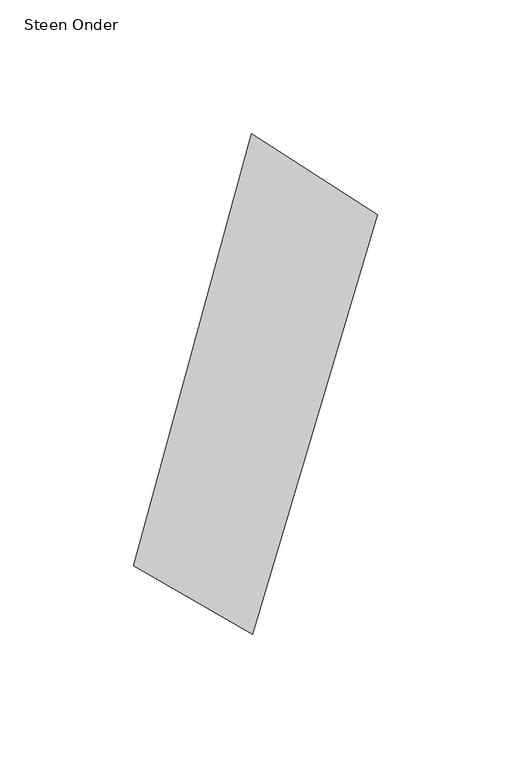
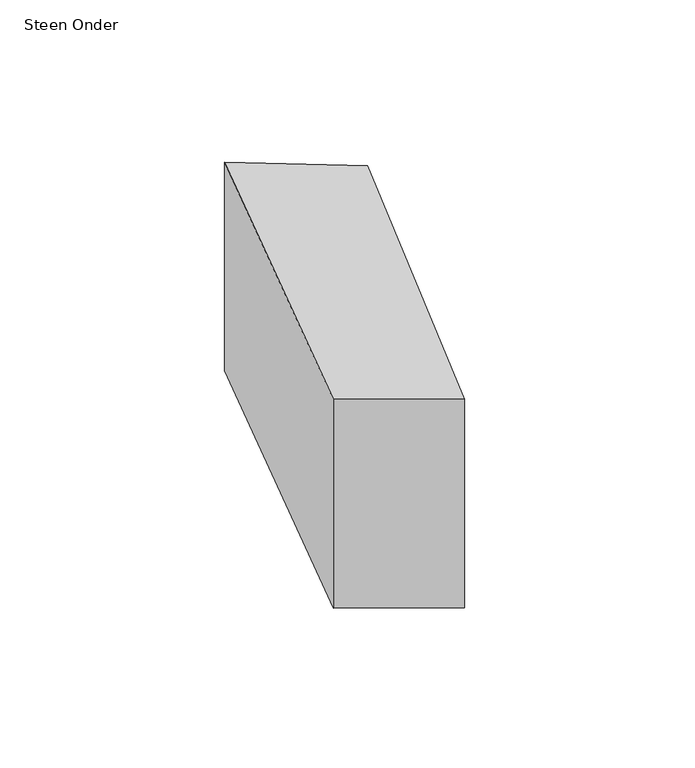
"""IFC4 building model written with IfcOpenShell, lengths in millimetres: proxy geometry, 00_GMA_steen_versie_4 : Steen Onder."""

import ifcopenshell
import ifcopenshell.guid

model = None  # the IFC model being written
_history = None  # IfcOwnerHistory: only IFC2X3 demands one
_inside = {}  # id of a spatial element -> (the spatial element, [elements in it])
_under = {}  # id of a project, library or spatial element -> (it, [spatial elements below it])
_declared = {}  # id of a project -> (the project, [libraries it declares])
_typed = {}  # id of a type object -> (the type object, [elements of that type])
_made_of = {}  # id of a material, layer set ... -> (it, [elements and type objects made of it])


def new_model(schema):
    """Start an empty IFC model of exactly this schema.

    Asked for "IFC4X3", IfcOpenShell would pick the latest addendum, in which some entities
    have other attributes; the version numbers below select the first issue.
    IFC2X3 requires an IfcOwnerHistory on every rooted entity: one is made here for all.
    """
    global model, _history
    if schema == "IFC4X3":
        model = ifcopenshell.file(schema_version=(4, 3, 0, 0))
    else:
        model = ifcopenshell.file(schema=schema)
    _inside.clear()
    _under.clear()
    _declared.clear()
    _typed.clear()
    _made_of.clear()
    _history = None
    if model.schema == "IFC2X3":
        org = make("IfcOrganization", Name="unknown")
        user = make(
            "IfcPersonAndOrganization",
            ThePerson=make("IfcPerson", FamilyName="unknown"),
            TheOrganization=org,
        )
        app = make(
            "IfcApplication",
            ApplicationDeveloper=org,
            Version="unknown",
            ApplicationFullName="unknown",
            ApplicationIdentifier="unknown",
        )
        _history = make(
            "IfcOwnerHistory",
            OwningUser=user,
            OwningApplication=app,
            ChangeAction="ADDED",
            CreationDate=0,
        )
    return model


def make(cls, **values):
    """One entity of the class cls with the attributes given. An attribute that is None is left unset."""
    return model.create_entity(
        cls, **{name: value for name, value in values.items() if value is not None}
    )


def rooted(cls, **values):
    """An entity with a GlobalId (a new one), such as an element, a storey or a relation."""
    return make(cls, GlobalId=ifcopenshell.guid.new(), OwnerHistory=_history, **values)


def si_unit(unit_type, name, prefix=None):
    """IfcSIUnit, for example si_unit("LENGTHUNIT", "METRE", prefix="MILLI")."""
    return make("IfcSIUnit", UnitType=unit_type, Prefix=prefix, Name=name)


def assignment(units):
    """IfcUnitAssignment: the units of a project."""
    return None if units is None else make("IfcUnitAssignment", Units=units)


def point(xyz):
    """IfcCartesianPoint."""
    return None if xyz is None else make("IfcCartesianPoint", Coordinates=xyz)


def direction(xyz):
    """IfcDirection."""
    return None if xyz is None else make("IfcDirection", DirectionRatios=xyz)


def frame(location, z_axis=None, x_axis=None):
    """IfcAxis2Placement3D, a coordinate frame: its origin and axes. An axis left out is left unset."""
    return make(
        "IfcAxis2Placement3D",
        Location=point(location),
        Axis=direction(z_axis),
        RefDirection=direction(x_axis),
    )


def origin():
    """The frame at (0, 0, 0) with its axes left unset."""
    return frame((0.0, 0.0, 0.0))


def origin_with_axes():
    """The frame at (0, 0, 0) with the z axis (0, 0, 1) and the x axis (1, 0, 0) written out."""
    return frame((0.0, 0.0, 0.0), z_axis=(0.0, 0.0, 1.0), x_axis=(1.0, 0.0, 0.0))


def place(relative_to, where):
    """IfcLocalPlacement: puts the frame where relative to a parent placement (None: the world)."""
    return make(
        "IfcLocalPlacement", PlacementRelTo=relative_to, RelativePlacement=where
    )


def context(
    kind, dimensions, precision=None, world=None, true_north=None, identifier=None
):
    """IfcGeometricRepresentationContext, for example the 3D "Model" context."""
    return make(
        "IfcGeometricRepresentationContext",
        ContextIdentifier=identifier,
        ContextType=kind,
        CoordinateSpaceDimension=dimensions,
        Precision=precision,
        WorldCoordinateSystem=world,
        TrueNorth=true_north,
    )


def project(units=None, contexts=None):
    """IfcProject with its units and contexts."""
    return rooted(
        "IfcProject",
        Name="project",
        RepresentationContexts=contexts,
        UnitsInContext=assignment(units),
    )


def spatial(cls, under=None, at=None, **own):
    """A site, building, storey or space (cls), placed at a placement, below another one or the project."""
    s = rooted(cls, ObjectPlacement=at, **own)
    if under is not None:
        _under.setdefault(under.id(), (under, []))[1].append(s)
    return s


def polyline(points):
    """IfcPolyline through the points."""
    return make("IfcPolyline", Points=[point(p) for p in points])


def outline(outer, holes=None, kind="AREA"):
    """IfcArbitraryClosedProfileDef: a profile drawn as a closed curve; with holes, ...WithVoids."""
    if holes is None:
        return make("IfcArbitraryClosedProfileDef", ProfileType=kind, OuterCurve=outer)
    return make(
        "IfcArbitraryProfileDefWithVoids",
        ProfileType=kind,
        OuterCurve=outer,
        InnerCurves=holes,
    )


def extrude(swept, where, along, depth):
    """IfcExtrudedAreaSolid: the profile swept, set in the frame where, extruded along a direction by depth."""
    return make(
        "IfcExtrudedAreaSolid",
        SweptArea=swept,
        Position=where,
        ExtrudedDirection=direction(along),
        Depth=depth,
    )


def shape(context_of_items, identifier, shape_type, items):
    """IfcShapeRepresentation: the items that make up one representation, for example the "Body"."""
    return make(
        "IfcShapeRepresentation",
        ContextOfItems=context_of_items,
        RepresentationIdentifier=identifier,
        RepresentationType=shape_type,
        Items=items,
    )


def source(mapping_origin, context_of_items, identifier, shape_type, items):
    """IfcRepresentationMap: a shape defined once, which mapped items show again and again."""
    return make(
        "IfcRepresentationMap",
        MappingOrigin=mapping_origin,
        MappedRepresentation=shape(context_of_items, identifier, shape_type, items),
    )


def transform(
    local_origin,
    x_axis=None,
    y_axis=None,
    z_axis=None,
    scale=None,
    scale2=None,
    scale3=None,
    uniform=True,
):
    """IfcCartesianTransformationOperator3D, or its non-uniform kind. x_axis, y_axis, z_axis: its Axis1, 2, 3."""
    if uniform:
        return make(
            "IfcCartesianTransformationOperator3D",
            Axis1=direction(x_axis),
            Axis2=direction(y_axis),
            LocalOrigin=point(local_origin),
            Scale=scale,
            Axis3=direction(z_axis),
        )
    return make(
        "IfcCartesianTransformationOperator3DnonUniform",
        Axis1=direction(x_axis),
        Axis2=direction(y_axis),
        LocalOrigin=point(local_origin),
        Scale=scale,
        Axis3=direction(z_axis),
        Scale2=scale2,
        Scale3=scale3,
    )


def mapped(mapping_source, mapping_target):
    """IfcMappedItem: shows the shape of a source again, moved by a transform."""
    return make(
        "IfcMappedItem", MappingSource=mapping_source, MappingTarget=mapping_target
    )


def made_of(thing, what):
    """Note that an element or type object is made of a material, layer set ...; save() writes the relation."""
    if what is not None:
        _made_of.setdefault(what.id(), (what, []))[1].append(thing)
    return thing


def element(
    cls,
    number,
    at=None,
    inside=None,
    cuts=None,
    type_object=None,
    material=None,
    context=None,
    identifier="Body",
    shape_type=None,
    held_by="IfcProductDefinitionShape",
    body=None,
    shapes=None,
    **own,
):
    """One element of the class cls, such as IfcWall. Its Tag is "e" and its number.

    at: its placement. inside: the storey or other place that contains it. cuts: it is an
    opening in that element (IfcRelVoidsElement). A single representation is given by context,
    identifier, shape_type and body (its items); several are given by shapes. held_by: the class
    of the entity that holds the representations. save() writes the other relations.
    """
    e = rooted(cls, Tag="e%d" % number, ObjectPlacement=at, **own)
    if body is not None:
        shapes = [shape(context, identifier, shape_type, body)]
    if shapes is not None:
        e.Representation = make(held_by, Representations=shapes)
    if inside is not None:
        _inside.setdefault(inside.id(), (inside, []))[1].append(e)
    if cuts is not None:
        rooted(
            "IfcRelVoidsElement", RelatingBuildingElement=cuts, RelatedOpeningElement=e
        )
    if type_object is not None:
        _typed.setdefault(type_object.id(), (type_object, []))[1].append(e)
    return made_of(e, material)


def aggregate(whole, parts):
    """IfcRelAggregates: a whole, such as a stair, and the parts it consists of."""
    return rooted("IfcRelAggregates", RelatingObject=whole, RelatedObjects=parts)


def save(model, path):
    """Write the relations noted so far, then the file.

    IfcRelAggregates (storeys below a building ...), IfcRelContainedInSpatialStructure (elements
    in a storey), IfcRelDefinesByType, IfcRelAssociatesMaterial and IfcRelDeclares: one each for
    every whole, place, type object, material and project.
    """
    for whole, parts in _under.values():
        aggregate(whole, parts)
    for where, things in _inside.values():
        rooted(
            "IfcRelContainedInSpatialStructure",
            RelatedElements=things,
            RelatingStructure=where,
        )
    for kind, things in _typed.values():
        rooted("IfcRelDefinesByType", RelatedObjects=things, RelatingType=kind)
    for what, things in _made_of.values():
        rooted("IfcRelAssociatesMaterial", RelatedObjects=things, RelatingMaterial=what)
    for by, libraries in _declared.values():
        rooted("IfcRelDeclares", RelatingContext=by, RelatedDefinitions=libraries)
    model.write(path)


def steen_onder_fb120837(model_context):
    return source(origin(), model_context, "Body", "SweptSolid", [
        extrude(outline(polyline([(123.9984619, 147.3054769), (77.1929147, -9.6177), (32.7327875, 15.9622446), (76.8290797, 177.6696463), (123.9984619, 147.3054769)])), origin_with_axes(), (0.0, 0.0, 1.0), 100.0),
    ])


if __name__ == "__main__":
    model = new_model("IFC4")
    model_context = context("Model", 3, world=origin())
    ifc_project = project(units=[si_unit("LENGTHUNIT", "METRE", prefix="MILLI")], contexts=[model_context])
    site = spatial("IfcSite", under=ifc_project)
    building = spatial("IfcBuilding", under=site)
    placement = place(None, origin())
    steen_onder_shape = steen_onder_fb120837(model_context)
    element("IfcBuildingElementProxy", 1, Name="00_GMA_steen_versie_4 : Steen Onder", ObjectType="00_GMA_steen_versie_4 : Steen Onder", at=placement, inside=building, context=model_context, shape_type="MappedRepresentation", body=[
        mapped(steen_onder_shape, transform((0.0, 0.0, 0.0), x_axis=(1.0, 0.0, 0.0), y_axis=(0.0, 1.0, 0.0), z_axis=(0.0, 0.0, 1.0))),
    ])
    save(model, "model.ifc")

# Revit data of these elements
# Type "00_GMA_steen_versie_4 : Steen Onder"
#   StootVoegHalfBoven [instance default] = 5 mm
#   StootVoegHalf [instance default] = 5 mm
#   StootVoegBreedteOnder = 10 mm
#   StootVoegBreedteBoven = 10 mm
#   Steendikte = 100 mm
#   LintVoegOnderHalf = 0 mm
#   LintVoegOnder = 0 mm
#   LintVoegBovenHalf = 5 mm
#   LintVoegBoven = 10 mm
#   materiaal = none
#   MateriaalVoeg = none
#   Default Elevation = 0
